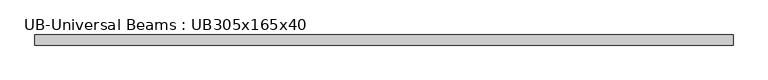
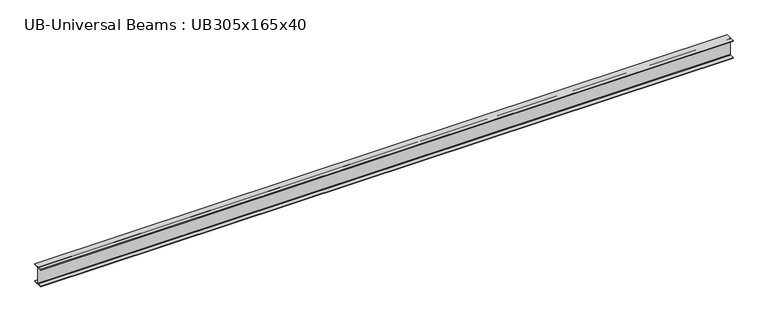
"""IFC4 building model written with IfcOpenShell, lengths in millimetres: member geometry, UB-Universal Beams : UB305x165x40."""

from ifc_helpers import new_model, si_unit, point, frame, frame_2d, origin, place, context, project, spatial, polyline, circle_curve, trimmed, segment, composite_curve, outline, extrude, source, transform, mapped, element, save


def ub_universal_beams_ub305x165x40_9e40c5b6(model_context):
    return source(origin(), model_context, "Body", "SweptSolid", [
        extrude(outline(composite_curve([segment(polyline([(82.5, -141.5), (82.5, -151.7), (-82.5, -151.7), (-82.5, -141.5), (-11.9, -141.5)]), True, "CONTINUOUS"), segment(trimmed(circle_curve(frame_2d((-11.9, -132.6)), 8.9), [point((-11.9, -141.5))], [point((-3.0, -132.6))], True, "CARTESIAN"), True, "CONTINUOUS"), segment(polyline([(-3.0, -132.6), (-3.0, 132.6)]), True, "CONTINUOUS"), segment(trimmed(circle_curve(frame_2d((-11.9, 132.6)), 8.9), [point((-3.0, 132.6))], [point((-11.9, 141.5))], True, "CARTESIAN"), True, "CONTINUOUS"), segment(polyline([(-11.9, 141.5), (-82.5, 141.5), (-82.5, 151.7), (82.5, 151.7), (82.5, 141.5), (11.9, 141.5)]), True, "CONTINUOUS"), segment(trimmed(circle_curve(frame_2d((11.9, 132.6)), 8.9), [point((11.9, 141.5))], [point((3.0, 132.6))], True, "CARTESIAN"), True, "CONTINUOUS"), segment(polyline([(3.0, 132.6), (3.0, -132.6)]), True, "CONTINUOUS"), segment(trimmed(circle_curve(frame_2d((11.9, -132.6)), 8.9), [point((3.0, -132.6))], [point((11.9, -141.5))], True, "CARTESIAN"), True, "CONTINUOUS"), segment(polyline([(11.9, -141.5), (82.5, -141.5)]), True, "CONTINUOUS")], self_intersect=False)), frame((-5682.6, 0.0, 0.0), z_axis=(1.0, 0.0, 0.0), x_axis=(0.0, 1.0, 0.0)), (0.0, 0.0, 1.0), 11365.2),
    ])


if __name__ == "__main__":
    model = new_model("IFC4")
    model_context = context("Model", 3, world=origin())
    ifc_project = project(units=[si_unit("LENGTHUNIT", "METRE", prefix="MILLI")], contexts=[model_context])
    site = spatial("IfcSite", under=ifc_project)
    building = spatial("IfcBuilding", under=site)
    placement = place(None, origin())
    ub_universal_beams_ub305x165x40_shape = ub_universal_beams_ub305x165x40_9e40c5b6(model_context)
    element("IfcMember", 1, ObjectType="UB-Universal Beams : UB305x165x40", at=placement, inside=building, context=model_context, shape_type="MappedRepresentation", body=[
        mapped(ub_universal_beams_ub305x165x40_shape, transform((0.0, 0.0, 0.0), x_axis=(1.0, 0.0, 0.0), y_axis=(0.0, 1.0, 0.0), z_axis=(0.0, 0.0, 1.0))),
    ])
    save(model, "model.ifc")

# Revit data of these elements
# Type "UB-Universal Beams : UB305x165x40"
#   Section Name Key = "UB305X165X40"
#   Width = 16.5 cm
#   Web Thickness = 0.6 cm
#   Web Fillet = 0.89 cm
#   Warping Constant = 164000.0 cm⁶
#   Torsional Moment of Inertia = 14.70 cm⁴
#   Section Area = 51.3 cm²
#   Plastic Modulus weak axis = 142.0 cm³
#   Plastic Modulus strong axis = 623.0 cm³
#   Nominal Weight = 40.2999 kgf/m
#   Moment of Inertia weak axis = 764.00 cm⁴
#   Moment of Inertia strong axis = 8503.00 cm⁴
#   Height = 30.34 cm
#   Flange Thickness = 1.02 cm
#   Elastic Modulus weak axis = 92.6 cm³
#   Elastic Modulus strong axis = 560.0 cm³
#   Centroid Vertical = 15.17 cm
#   Centroid Horizontal = 8.25 cm
#   Bolt Spacing = 9.0 cm
#   Length [instance default] = 1500 mm
#   Structural Material [instance default] = Metal - Steel 43-275
#   Type Comments = ""
#   Assembly Code = ""
# Element 1 (IfcMember, "UB-Universal Beams : UB305x165x40")
#   Materials on its faces: "Metal - Steel 43-275"
# Materials
#   "Metal - Steel 43-275": class "Metal", colour RGB 247 247 247, transparency 0, Cost = 0
